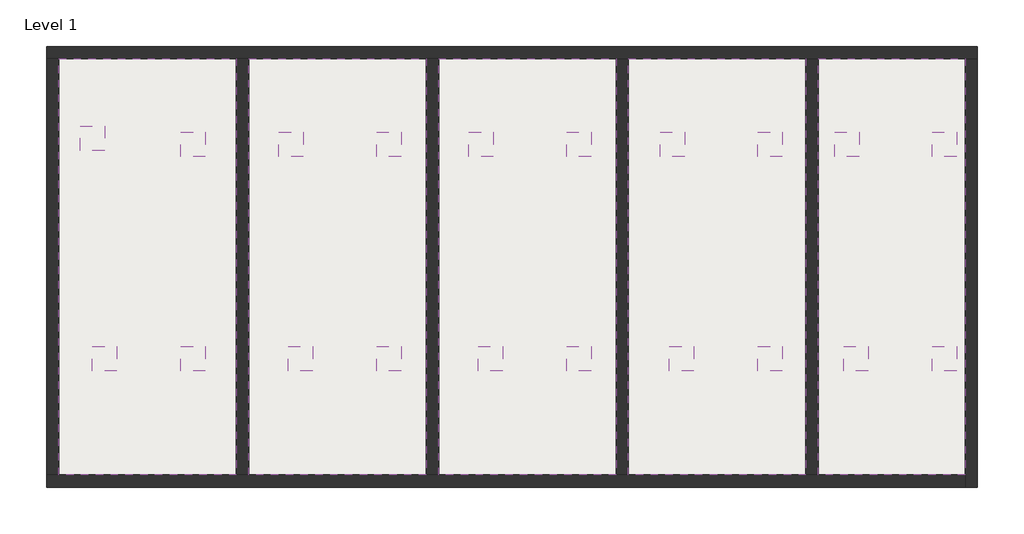
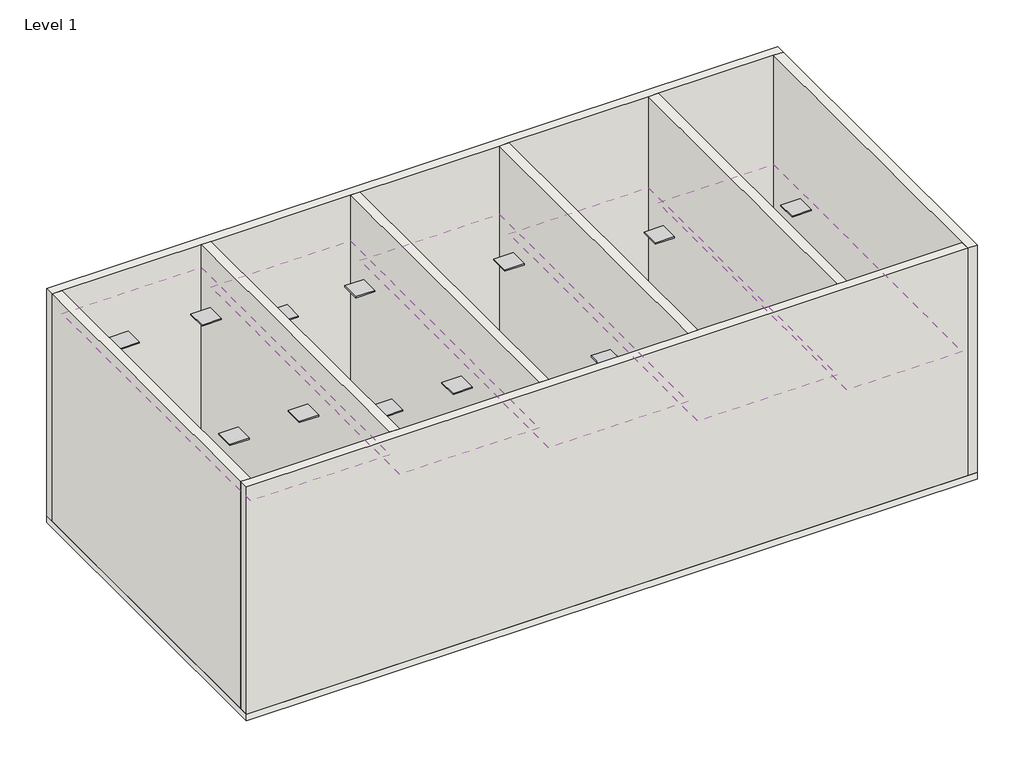
# One storey: 20 light fixtures, 8 walls, 5 coverings, 1 slab.
"""IFC4 building model written with IfcOpenShell, lengths in millimetres."""

import ifcopenshell
import ifcopenshell.guid

model = None  # the IFC model being written
_history = None  # IfcOwnerHistory: only IFC2X3 demands one
_inside = {}  # id of a spatial element -> (the spatial element, [elements in it])
_under = {}  # id of a project, library or spatial element -> (it, [spatial elements below it])
_declared = {}  # id of a project -> (the project, [libraries it declares])
_typed = {}  # id of a type object -> (the type object, [elements of that type])
_made_of = {}  # id of a material, layer set ... -> (it, [elements and type objects made of it])


def new_model(schema):
    """Start an empty IFC model of exactly this schema.

    Asked for "IFC4X3", IfcOpenShell would pick the latest addendum, in which some entities
    have other attributes; the version numbers below select the first issue.
    IFC2X3 requires an IfcOwnerHistory on every rooted entity: one is made here for all.
    """
    global model, _history
    if schema == "IFC4X3":
        model = ifcopenshell.file(schema_version=(4, 3, 0, 0))
    else:
        model = ifcopenshell.file(schema=schema)
    _inside.clear()
    _under.clear()
    _declared.clear()
    _typed.clear()
    _made_of.clear()
    _history = None
    if model.schema == "IFC2X3":
        org = make("IfcOrganization", Name="unknown")
        user = make(
            "IfcPersonAndOrganization",
            ThePerson=make("IfcPerson", FamilyName="unknown"),
            TheOrganization=org,
        )
        app = make(
            "IfcApplication",
            ApplicationDeveloper=org,
            Version="unknown",
            ApplicationFullName="unknown",
            ApplicationIdentifier="unknown",
        )
        _history = make(
            "IfcOwnerHistory",
            OwningUser=user,
            OwningApplication=app,
            ChangeAction="ADDED",
            CreationDate=0,
        )
    return model


def make(cls, **values):
    """One entity of the class cls with the attributes given. An attribute that is None is left unset."""
    return model.create_entity(
        cls, **{name: value for name, value in values.items() if value is not None}
    )


def rooted(cls, **values):
    """An entity with a GlobalId (a new one), such as an element, a storey or a relation."""
    return make(cls, GlobalId=ifcopenshell.guid.new(), OwnerHistory=_history, **values)


def si_unit(unit_type, name, prefix=None):
    """IfcSIUnit, for example si_unit("LENGTHUNIT", "METRE", prefix="MILLI")."""
    return make("IfcSIUnit", UnitType=unit_type, Prefix=prefix, Name=name)


def assignment(units):
    """IfcUnitAssignment: the units of a project."""
    return None if units is None else make("IfcUnitAssignment", Units=units)


def point(xyz):
    """IfcCartesianPoint."""
    return None if xyz is None else make("IfcCartesianPoint", Coordinates=xyz)


def direction(xyz):
    """IfcDirection."""
    return None if xyz is None else make("IfcDirection", DirectionRatios=xyz)


def frame(location, z_axis=None, x_axis=None):
    """IfcAxis2Placement3D, a coordinate frame: its origin and axes. An axis left out is left unset."""
    return make(
        "IfcAxis2Placement3D",
        Location=point(location),
        Axis=direction(z_axis),
        RefDirection=direction(x_axis),
    )


def origin():
    """The frame at (0, 0, 0) with its axes left unset."""
    return frame((0.0, 0.0, 0.0))


def origin_with_axes():
    """The frame at (0, 0, 0) with the z axis (0, 0, 1) and the x axis (1, 0, 0) written out."""
    return frame((0.0, 0.0, 0.0), z_axis=(0.0, 0.0, 1.0), x_axis=(1.0, 0.0, 0.0))


def place(relative_to, where):
    """IfcLocalPlacement: puts the frame where relative to a parent placement (None: the world)."""
    return make(
        "IfcLocalPlacement", PlacementRelTo=relative_to, RelativePlacement=where
    )


def context(
    kind, dimensions, precision=None, world=None, true_north=None, identifier=None
):
    """IfcGeometricRepresentationContext, for example the 3D "Model" context."""
    return make(
        "IfcGeometricRepresentationContext",
        ContextIdentifier=identifier,
        ContextType=kind,
        CoordinateSpaceDimension=dimensions,
        Precision=precision,
        WorldCoordinateSystem=world,
        TrueNorth=true_north,
    )


def project(units=None, contexts=None):
    """IfcProject with its units and contexts."""
    return rooted(
        "IfcProject",
        Name="project",
        RepresentationContexts=contexts,
        UnitsInContext=assignment(units),
    )


def spatial(cls, under=None, at=None, **own):
    """A site, building, storey or space (cls), placed at a placement, below another one or the project."""
    s = rooted(cls, ObjectPlacement=at, **own)
    if under is not None:
        _under.setdefault(under.id(), (under, []))[1].append(s)
    return s


def polyline(points):
    """IfcPolyline through the points."""
    return make("IfcPolyline", Points=[point(p) for p in points])


def outline(outer, holes=None, kind="AREA"):
    """IfcArbitraryClosedProfileDef: a profile drawn as a closed curve; with holes, ...WithVoids."""
    if holes is None:
        return make("IfcArbitraryClosedProfileDef", ProfileType=kind, OuterCurve=outer)
    return make(
        "IfcArbitraryProfileDefWithVoids",
        ProfileType=kind,
        OuterCurve=outer,
        InnerCurves=holes,
    )


def extrude(swept, where, along, depth):
    """IfcExtrudedAreaSolid: the profile swept, set in the frame where, extruded along a direction by depth."""
    return make(
        "IfcExtrudedAreaSolid",
        SweptArea=swept,
        Position=where,
        ExtrudedDirection=direction(along),
        Depth=depth,
    )


def faces_of(points, faces, orient=None, outer=None):
    """IfcFace entities. A face is a list of loops; a loop is a list of indices into points, from 0.

    orient and outer hold one flag for each loop. By default every Orientation is true, the
    first loop of a face is its IfcFaceOuterBound and the others are IfcFaceBound.
    """
    made = []
    for i, loops in enumerate(faces):
        bounds = []
        for j, loop in enumerate(loops):
            is_outer = j == 0 if outer is None else outer[i][j]
            bounds.append(
                make(
                    "IfcFaceOuterBound" if is_outer else "IfcFaceBound",
                    Bound=make("IfcPolyLoop", Polygon=[points[k] for k in loop]),
                    Orientation=True if orient is None else orient[i][j],
                )
            )
        made.append(make("IfcFace", Bounds=bounds))
    return made


def faceted_brep(points, faces, orient=None, outer=None, voids=None):
    """IfcFacetedBrep: a solid bounded by flat faces; with voids (closed shells), ...WithVoids."""
    shared = [point(p) for p in points]
    hull = make("IfcClosedShell", CfsFaces=faces_of(shared, faces, orient, outer))
    if voids is None:
        return make("IfcFacetedBrep", Outer=hull)
    return make(
        "IfcFacetedBrepWithVoids",
        Outer=hull,
        Voids=[
            make(cls, CfsFaces=faces_of(shared, fs, o, b)) for cls, fs, o, b in voids
        ],
    )


def shape(context_of_items, identifier, shape_type, items):
    """IfcShapeRepresentation: the items that make up one representation, for example the "Body"."""
    return make(
        "IfcShapeRepresentation",
        ContextOfItems=context_of_items,
        RepresentationIdentifier=identifier,
        RepresentationType=shape_type,
        Items=items,
    )


def source(mapping_origin, context_of_items, identifier, shape_type, items):
    """IfcRepresentationMap: a shape defined once, which mapped items show again and again."""
    return make(
        "IfcRepresentationMap",
        MappingOrigin=mapping_origin,
        MappedRepresentation=shape(context_of_items, identifier, shape_type, items),
    )


def transform(
    local_origin,
    x_axis=None,
    y_axis=None,
    z_axis=None,
    scale=None,
    scale2=None,
    scale3=None,
    uniform=True,
):
    """IfcCartesianTransformationOperator3D, or its non-uniform kind. x_axis, y_axis, z_axis: its Axis1, 2, 3."""
    if uniform:
        return make(
            "IfcCartesianTransformationOperator3D",
            Axis1=direction(x_axis),
            Axis2=direction(y_axis),
            LocalOrigin=point(local_origin),
            Scale=scale,
            Axis3=direction(z_axis),
        )
    return make(
        "IfcCartesianTransformationOperator3DnonUniform",
        Axis1=direction(x_axis),
        Axis2=direction(y_axis),
        LocalOrigin=point(local_origin),
        Scale=scale,
        Axis3=direction(z_axis),
        Scale2=scale2,
        Scale3=scale3,
    )


def mapped(mapping_source, mapping_target):
    """IfcMappedItem: shows the shape of a source again, moved by a transform."""
    return make(
        "IfcMappedItem", MappingSource=mapping_source, MappingTarget=mapping_target
    )


def made_of(thing, what):
    """Note that an element or type object is made of a material, layer set ...; save() writes the relation."""
    if what is not None:
        _made_of.setdefault(what.id(), (what, []))[1].append(thing)
    return thing


def element(
    cls,
    number,
    at=None,
    inside=None,
    cuts=None,
    type_object=None,
    material=None,
    context=None,
    identifier="Body",
    shape_type=None,
    held_by="IfcProductDefinitionShape",
    body=None,
    shapes=None,
    **own,
):
    """One element of the class cls, such as IfcWall. Its Tag is "e" and its number.

    at: its placement. inside: the storey or other place that contains it. cuts: it is an
    opening in that element (IfcRelVoidsElement). A single representation is given by context,
    identifier, shape_type and body (its items); several are given by shapes. held_by: the class
    of the entity that holds the representations. save() writes the other relations.
    """
    e = rooted(cls, Tag="e%d" % number, ObjectPlacement=at, **own)
    if body is not None:
        shapes = [shape(context, identifier, shape_type, body)]
    if shapes is not None:
        e.Representation = make(held_by, Representations=shapes)
    if inside is not None:
        _inside.setdefault(inside.id(), (inside, []))[1].append(e)
    if cuts is not None:
        rooted(
            "IfcRelVoidsElement", RelatingBuildingElement=cuts, RelatedOpeningElement=e
        )
    if type_object is not None:
        _typed.setdefault(type_object.id(), (type_object, []))[1].append(e)
    return made_of(e, material)


def aggregate(whole, parts):
    """IfcRelAggregates: a whole, such as a stair, and the parts it consists of."""
    return rooted("IfcRelAggregates", RelatingObject=whole, RelatedObjects=parts)


def save(model, path):
    """Write the relations noted so far, then the file.

    IfcRelAggregates (storeys below a building ...), IfcRelContainedInSpatialStructure (elements
    in a storey), IfcRelDefinesByType, IfcRelAssociatesMaterial and IfcRelDeclares: one each for
    every whole, place, type object, material and project.
    """
    for whole, parts in _under.values():
        aggregate(whole, parts)
    for where, things in _inside.values():
        rooted(
            "IfcRelContainedInSpatialStructure",
            RelatedElements=things,
            RelatingStructure=where,
        )
    for kind, things in _typed.values():
        rooted("IfcRelDefinesByType", RelatedObjects=things, RelatingType=kind)
    for what, things in _made_of.values():
        rooted("IfcRelAssociatesMaterial", RelatedObjects=things, RelatingMaterial=what)
    for by, libraries in _declared.values():
        rooted("IfcRelDeclares", RelatingContext=by, RelatedDefinitions=libraries)
    model.write(path)


def downlight_downlight_20077eaa(model_context):
    return source(origin(), model_context, "Body", "SweptSolid", [
        extrude(outline(polyline([(200.0, -200.0), (-200.0, -200.0), (-200.0, 200.0), (200.0, 200.0), (200.0, -200.0)])), frame((0.0, 0.0, -4.6872227), z_axis=(0.0, 0.0, 1.0), x_axis=(1.0, 0.0, 0.0)), (0.0, 0.0, 1.0), 24.9370919),
    ])


model = new_model("IFC4")

# Units and contexts
model_context = context("Model", 3, world=origin())
ifc_project = project(units=[si_unit("LENGTHUNIT", "METRE", prefix="MILLI")], contexts=[model_context])

# Site, building, storey
site = spatial("IfcSite", under=ifc_project)
building = spatial("IfcBuilding", under=site)
storey = spatial("IfcBuildingStorey", under=building, Name="Level 1", Elevation=0.0)

# Coverings
placement = place(None, origin())
element("IfcCovering", 1, ObjectType="600 x 600mm Grid", at=placement, inside=storey, context=model_context, shape_type="SweptSolid", body=[
    extrude(outline(polyline([(4711.6370984, -2494.7382368), (4711.6370984, 4305.2617632), (7111.6370984, 4305.2617632), (7111.6370984, -2494.7382368), (4711.6370984, -2494.7382368)])), frame((0.0, 0.0, 2600.0), z_axis=(0.0, 0.0, 1.0), x_axis=(1.0, 0.0, 0.0)), (0.0, 0.0, 1.0), 52.0),
])
element("IfcCovering", 2, ObjectType="600 x 600mm Grid", at=placement, inside=storey, context=model_context, shape_type="SweptSolid", body=[
    extrude(outline(polyline([(1611.6370984, -2494.7382368), (1611.6370984, 4305.2617632), (4511.6370984, 4305.2617632), (4511.6370984, -2494.7382368), (1611.6370984, -2494.7382368)])), frame((0.0, 0.0, 3000.0), z_axis=(0.0, 0.0, 1.0), x_axis=(1.0, 0.0, 0.0)), (0.0, 0.0, 1.0), 52.0),
])
element("IfcCovering", 3, ObjectType="600 x 600mm Grid", at=placement, inside=storey, context=model_context, shape_type="SweptSolid", body=[
    extrude(outline(polyline([(-1488.3629016, -2494.7382368), (-1488.3629016, 4305.2617632), (1411.6370984, 4305.2617632), (1411.6370984, -2494.7382368), (-1488.3629016, -2494.7382368)])), frame((0.0, 0.0, 3500.0), z_axis=(0.0, 0.0, 1.0), x_axis=(1.0, 0.0, 0.0)), (0.0, 0.0, 1.0), 52.0),
])
element("IfcCovering", 4, ObjectType="600 x 600mm Grid", at=placement, inside=storey, context=model_context, shape_type="SweptSolid", body=[
    extrude(outline(polyline([(-4588.3629016, -2494.7382368), (-4588.3629016, 4305.2617632), (-1688.3629016, 4305.2617632), (-1688.3629016, -2494.7382368), (-4588.3629016, -2494.7382368)])), frame((0.0, 0.0, 4000.0), z_axis=(0.0, 0.0, 1.0), x_axis=(1.0, 0.0, 0.0)), (0.0, 0.0, 1.0), 52.0),
])
element("IfcCovering", 5, ObjectType="600 x 600mm Grid", at=placement, inside=storey, context=model_context, shape_type="SweptSolid", body=[
    extrude(outline(polyline([(-7688.3629016, 4305.2617632), (-4788.3629016, 4305.2617632), (-4788.3629016, -2494.7382368), (-7688.3629016, -2494.7382368), (-7688.3629016, 4305.2617632)])), frame((0.0, 0.0, 4500.0), z_axis=(0.0, 0.0, 1.0), x_axis=(1.0, 0.0, 0.0)), (0.0, 0.0, 1.0), 52.0),
])

# Light fixtures
downlight_downlight_shape = downlight_downlight_20077eaa(model_context)
element("IfcLightFixture", 6, ObjectType="Downlight : Downlight", at=placement, inside=storey, context=model_context, shape_type="MappedRepresentation", body=[
    mapped(downlight_downlight_shape, transform((-7138.3629016, 3005.2617632, 4500.0), x_axis=(1.0, 0.0, 0.0), y_axis=(0.0, 1.0, 0.0), z_axis=(0.0, 0.0, 1.0))),
])
element("IfcLightFixture", 7, ObjectType="Downlight : Downlight", at=placement, inside=storey, context=model_context, shape_type="MappedRepresentation", body=[
    mapped(downlight_downlight_shape, transform((-5493.1629016, 2905.2617632, 4500.0), x_axis=(1.0, 0.0, 0.0), y_axis=(0.0, 1.0, 0.0), z_axis=(0.0, 0.0, 1.0))),
])
element("IfcLightFixture", 8, ObjectType="Downlight : Downlight", at=placement, inside=storey, context=model_context, shape_type="MappedRepresentation", body=[
    mapped(downlight_downlight_shape, transform((-5493.1629016, -599.5382368, 4500.0), x_axis=(1.0, 0.0, 0.0), y_axis=(0.0, 1.0, 0.0), z_axis=(0.0, 0.0, 1.0))),
])
element("IfcLightFixture", 9, ObjectType="Downlight : Downlight", at=placement, inside=storey, context=model_context, shape_type="MappedRepresentation", body=[
    mapped(downlight_downlight_shape, transform((-6938.3629016, -599.5382368, 4500.0), x_axis=(1.0, 0.0, 0.0), y_axis=(0.0, 1.0, 0.0), z_axis=(0.0, 0.0, 1.0))),
])
element("IfcLightFixture", 10, ObjectType="Downlight : Downlight", at=placement, inside=storey, context=model_context, shape_type="MappedRepresentation", body=[
    mapped(downlight_downlight_shape, transform((-3893.1629016, 2905.2617632, 4000.0), x_axis=(1.0, 0.0, 0.0), y_axis=(0.0, 1.0, 0.0), z_axis=(0.0, 0.0, 1.0))),
])
element("IfcLightFixture", 11, ObjectType="Downlight : Downlight", at=placement, inside=storey, context=model_context, shape_type="MappedRepresentation", body=[
    mapped(downlight_downlight_shape, transform((-2297.9629016, 2905.2617632, 4000.0), x_axis=(1.0, 0.0, 0.0), y_axis=(0.0, 1.0, 0.0), z_axis=(0.0, 0.0, 1.0))),
])
element("IfcLightFixture", 12, ObjectType="Downlight : Downlight", at=placement, inside=storey, context=model_context, shape_type="MappedRepresentation", body=[
    mapped(downlight_downlight_shape, transform((-2297.9629016, -599.5382368, 4000.0), x_axis=(1.0, 0.0, 0.0), y_axis=(0.0, 1.0, 0.0), z_axis=(0.0, 0.0, 1.0))),
])
element("IfcLightFixture", 13, ObjectType="Downlight : Downlight", at=placement, inside=storey, context=model_context, shape_type="MappedRepresentation", body=[
    mapped(downlight_downlight_shape, transform((-3743.1629016, -599.5382368, 4000.0), x_axis=(1.0, 0.0, 0.0), y_axis=(0.0, 1.0, 0.0), z_axis=(0.0, 0.0, 1.0))),
])
element("IfcLightFixture", 14, ObjectType="Downlight : Downlight", at=placement, inside=storey, context=model_context, shape_type="MappedRepresentation", body=[
    mapped(downlight_downlight_shape, transform((-790.9030237, 2905.2617632, 3500.0), x_axis=(1.0, 0.0, 0.0), y_axis=(0.0, 1.0, 0.0), z_axis=(0.0, 0.0, 1.0))),
])
element("IfcLightFixture", 15, ObjectType="Downlight : Downlight", at=placement, inside=storey, context=model_context, shape_type="MappedRepresentation", body=[
    mapped(downlight_downlight_shape, transform((804.2969763, 2905.2617632, 3500.0), x_axis=(1.0, 0.0, 0.0), y_axis=(0.0, 1.0, 0.0), z_axis=(0.0, 0.0, 1.0))),
])
element("IfcLightFixture", 16, ObjectType="Downlight : Downlight", at=placement, inside=storey, context=model_context, shape_type="MappedRepresentation", body=[
    mapped(downlight_downlight_shape, transform((804.2969763, -599.5382368, 3500.0), x_axis=(1.0, 0.0, 0.0), y_axis=(0.0, 1.0, 0.0), z_axis=(0.0, 0.0, 1.0))),
])
element("IfcLightFixture", 17, ObjectType="Downlight : Downlight", at=placement, inside=storey, context=model_context, shape_type="MappedRepresentation", body=[
    mapped(downlight_downlight_shape, transform((-640.9030237, -599.5382368, 3500.0), x_axis=(1.0, 0.0, 0.0), y_axis=(0.0, 1.0, 0.0), z_axis=(0.0, 0.0, 1.0))),
])
element("IfcLightFixture", 18, ObjectType="Downlight : Downlight", at=placement, inside=storey, context=model_context, shape_type="MappedRepresentation", body=[
    mapped(downlight_downlight_shape, transform((2331.8395219, 2905.2617632, 3000.0), x_axis=(1.0, 0.0, 0.0), y_axis=(0.0, 1.0, 0.0), z_axis=(0.0, 0.0, 1.0))),
])
element("IfcLightFixture", 19, ObjectType="Downlight : Downlight", at=placement, inside=storey, context=model_context, shape_type="MappedRepresentation", body=[
    mapped(downlight_downlight_shape, transform((3927.0395219, 2905.2617632, 3000.0), x_axis=(1.0, 0.0, 0.0), y_axis=(0.0, 1.0, 0.0), z_axis=(0.0, 0.0, 1.0))),
])
element("IfcLightFixture", 20, ObjectType="Downlight : Downlight", at=placement, inside=storey, context=model_context, shape_type="MappedRepresentation", body=[
    mapped(downlight_downlight_shape, transform((3927.0395219, -599.5382368, 3000.0), x_axis=(1.0, 0.0, 0.0), y_axis=(0.0, 1.0, 0.0), z_axis=(0.0, 0.0, 1.0))),
])
element("IfcLightFixture", 21, ObjectType="Downlight : Downlight", at=placement, inside=storey, context=model_context, shape_type="MappedRepresentation", body=[
    mapped(downlight_downlight_shape, transform((2481.8395219, -599.5382368, 3000.0), x_axis=(1.0, 0.0, 0.0), y_axis=(0.0, 1.0, 0.0), z_axis=(0.0, 0.0, 1.0))),
])
element("IfcLightFixture", 22, ObjectType="Downlight : Downlight", at=placement, inside=storey, context=model_context, shape_type="MappedRepresentation", body=[
    mapped(downlight_downlight_shape, transform((5177.9874108, 2905.2617632, 2600.0), x_axis=(1.0, 0.0, 0.0), y_axis=(0.0, 1.0, 0.0), z_axis=(0.0, 0.0, 1.0))),
])
element("IfcLightFixture", 23, ObjectType="Downlight : Downlight", at=placement, inside=storey, context=model_context, shape_type="MappedRepresentation", body=[
    mapped(downlight_downlight_shape, transform((6773.1874108, 2905.2617632, 2600.0), x_axis=(1.0, 0.0, 0.0), y_axis=(0.0, 1.0, 0.0), z_axis=(0.0, 0.0, 1.0))),
])
element("IfcLightFixture", 24, ObjectType="Downlight : Downlight", at=placement, inside=storey, context=model_context, shape_type="MappedRepresentation", body=[
    mapped(downlight_downlight_shape, transform((6773.1874108, -599.5382368, 2600.0), x_axis=(1.0, 0.0, 0.0), y_axis=(0.0, 1.0, 0.0), z_axis=(0.0, 0.0, 1.0))),
])
element("IfcLightFixture", 25, ObjectType="Downlight : Downlight", at=placement, inside=storey, context=model_context, shape_type="MappedRepresentation", body=[
    mapped(downlight_downlight_shape, transform((5327.9874108, -599.5382368, 2600.0), x_axis=(1.0, 0.0, 0.0), y_axis=(0.0, 1.0, 0.0), z_axis=(0.0, 0.0, 1.0))),
])

# Slab
element("IfcSlab", 26, ObjectType="Generic 150mm", at=placement, inside=storey, context=model_context, shape_type="SweptSolid", body=[
    extrude(outline(polyline([(7311.6370984, 4505.2617632), (7311.6370984, -2694.7382368), (-7888.3629016, -2694.7382368), (-7888.3629016, 4505.2617632), (7311.6370984, 4505.2617632)])), frame((0.0, 0.0, -150.0), z_axis=(0.0, 0.0, 1.0), x_axis=(1.0, 0.0, 0.0)), (0.0, 0.0, 1.0), 150.0),
])

# Walls
element("IfcWall", 27, ObjectType="Generic - 200mm", at=placement, inside=storey, context=model_context, shape_type="Brep", body=[
    faceted_brep([(-7888.3629016, 4305.2617632, 0.0), (-7688.3629016, 4305.2617632, 0.0), (-4788.3629016, 4305.2617632, 0.0), (-4588.3629016, 4305.2617632, 0.0), (-1688.3629016, 4305.2617632, 0.0), (-1488.3629016, 4305.2617632, 0.0), (1411.6370984, 4305.2617632, 0.0), (1611.6370984, 4305.2617632, 0.0), (4511.6370984, 4305.2617632, 0.0), (4711.6370984, 4305.2617632, 0.0), (7111.6370984, 4305.2617632, 0.0), (7311.6370984, 4305.2617632, 0.0), (7311.6370984, 4305.2617632, 5000.0), (7111.6370984, 4305.2617632, 5000.0), (4711.6370984, 4305.2617632, 5000.0), (4511.6370984, 4305.2617632, 5000.0), (1611.6370984, 4305.2617632, 5000.0), (1411.6370984, 4305.2617632, 5000.0), (-1488.3629016, 4305.2617632, 5000.0), (-1688.3629016, 4305.2617632, 5000.0), (-4588.3629016, 4305.2617632, 5000.0), (-4788.3629016, 4305.2617632, 5000.0), (-7688.3629016, 4305.2617632, 5000.0), (-7888.3629016, 4305.2617632, 5000.0), (-7888.3629016, 4505.2617632, 0.0), (-7888.3629016, 4505.2617632, 5000.0), (7311.6370984, 4505.2617632, 5000.0), (7311.6370984, 4505.2617632, 0.0)], [[[0, 1, 2, 3, 4, 5, 6, 7, 8, 9, 10, 11, 12, 13, 14, 15, 16, 17, 18, 19, 20, 21, 22, 23]], [[24, 25, 26, 27]], [[11, 10, 9, 8, 7, 6, 5, 4, 3, 2, 1, 0, 24, 27]], [[23, 22, 21, 20, 19, 18, 17, 16, 15, 14, 13, 12, 26, 25]], [[12, 11, 27, 26]], [[0, 23, 25, 24]]]),
])
element("IfcWall", 28, ObjectType="Generic - 200mm", at=placement, inside=storey, context=model_context, shape_type="Brep", body=[
    faceted_brep([(7111.6370984, 4305.2617632, 0.0), (7111.6370984, -2494.7382368, 0.0), (7111.6370984, -2694.7382368, 0.0), (7111.6370984, -2694.7382368, 5000.0), (7111.6370984, -2494.7382368, 5000.0), (7111.6370984, 4305.2617632, 5000.0), (7311.6370984, 4305.2617632, 0.0), (7311.6370984, 4305.2617632, 5000.0), (7311.6370984, -2694.7382368, 5000.0), (7311.6370984, -2694.7382368, 0.0)], [[[0, 1, 2, 3, 4, 5]], [[6, 7, 8, 9]], [[2, 1, 0, 6, 9]], [[5, 4, 3, 8, 7]], [[0, 5, 7, 6]], [[3, 2, 9, 8]]]),
])
element("IfcWall", 29, ObjectType="Generic - 200mm", at=placement, inside=storey, context=model_context, shape_type="Brep", body=[
    faceted_brep([(7111.6370984, -2494.7382368, 0.0), (4711.6370984, -2494.7382368, 0.0), (4511.6370984, -2494.7382368, 0.0), (1611.6370984, -2494.7382368, 0.0), (1411.6370984, -2494.7382368, 0.0), (-1488.3629016, -2494.7382368, 0.0), (-1688.3629016, -2494.7382368, 0.0), (-4588.3629016, -2494.7382368, 0.0), (-4788.3629016, -2494.7382368, 0.0), (-7688.3629016, -2494.7382368, 0.0), (-7888.3629016, -2494.7382368, 0.0), (-7888.3629016, -2494.7382368, 5000.0), (-7688.3629016, -2494.7382368, 5000.0), (-4788.3629016, -2494.7382368, 5000.0), (-4588.3629016, -2494.7382368, 5000.0), (-1688.3629016, -2494.7382368, 5000.0), (-1488.3629016, -2494.7382368, 5000.0), (1411.6370984, -2494.7382368, 5000.0), (1611.6370984, -2494.7382368, 5000.0), (4511.6370984, -2494.7382368, 5000.0), (4711.6370984, -2494.7382368, 5000.0), (7111.6370984, -2494.7382368, 5000.0), (7111.6370984, -2694.7382368, 0.0), (7111.6370984, -2694.7382368, 5000.0), (-7888.3629016, -2694.7382368, 5000.0), (-7888.3629016, -2694.7382368, 0.0)], [[[0, 1, 2, 3, 4, 5, 6, 7, 8, 9, 10, 11, 12, 13, 14, 15, 16, 17, 18, 19, 20, 21]], [[22, 23, 24, 25]], [[10, 9, 8, 7, 6, 5, 4, 3, 2, 1, 0, 22, 25]], [[21, 20, 19, 18, 17, 16, 15, 14, 13, 12, 11, 24, 23]], [[0, 21, 23, 22]], [[11, 10, 25, 24]]]),
])
element("IfcWall", 30, ObjectType="Generic - 200mm", at=placement, inside=storey, context=model_context, shape_type="SweptSolid", body=[
    extrude(outline(polyline([(-7688.3629016, 4305.2617632), (-7688.3629016, -2494.7382368), (-7888.3629016, -2494.7382368), (-7888.3629016, 4305.2617632), (-7688.3629016, 4305.2617632)])), origin_with_axes(), (0.0, 0.0, 1.0), 5000.0),
])
element("IfcWall", 31, ObjectType="Generic - 200mm", at=placement, inside=storey, context=model_context, shape_type="SweptSolid", body=[
    extrude(outline(polyline([(-4788.3629016, -2494.7382368), (-4788.3629016, 4305.2617632), (-4588.3629016, 4305.2617632), (-4588.3629016, -2494.7382368), (-4788.3629016, -2494.7382368)])), origin_with_axes(), (0.0, 0.0, 1.0), 5000.0),
])
element("IfcWall", 32, ObjectType="Generic - 200mm", at=placement, inside=storey, context=model_context, shape_type="SweptSolid", body=[
    extrude(outline(polyline([(-1688.3629016, -2494.7382368), (-1688.3629016, 4305.2617632), (-1488.3629016, 4305.2617632), (-1488.3629016, -2494.7382368), (-1688.3629016, -2494.7382368)])), origin_with_axes(), (0.0, 0.0, 1.0), 5000.0),
])
element("IfcWall", 33, ObjectType="Generic - 200mm", at=placement, inside=storey, context=model_context, shape_type="SweptSolid", body=[
    extrude(outline(polyline([(1411.6370984, -2494.7382368), (1411.6370984, 4305.2617632), (1611.6370984, 4305.2617632), (1611.6370984, -2494.7382368), (1411.6370984, -2494.7382368)])), origin_with_axes(), (0.0, 0.0, 1.0), 5000.0),
])
element("IfcWall", 34, ObjectType="Generic - 200mm", at=placement, inside=storey, context=model_context, shape_type="SweptSolid", body=[
    extrude(outline(polyline([(4511.6370984, -2494.7382368), (4511.6370984, 4305.2617632), (4711.6370984, 4305.2617632), (4711.6370984, -2494.7382368), (4511.6370984, -2494.7382368)])), origin_with_axes(), (0.0, 0.0, 1.0), 5000.0),
])

save(model, "model.ifc")

# Revit data of these elements
# Project information
#   Project Issue Date = "Issue Date"
#   Project Status = "Project Status"
#   Client Name = "Owner"
#   Project Address = "Enter address here"
#   Project Name = "Project Name"
#   Project Number = "0001"
# Type "600 x 600mm Grid"
#   built-in parameter 1002203 = 1 (stored number, unit not read)
#   built-in parameter 1002202 = 1 (stored number, unit not read)
#   Layers, outside or top first: 0.036 m "Default" (function 1); 0.016 m "Ceiling Tile 600 x 600" (function 5)
# Type "Downlight : Downlight"
#   Default Elevation = 0
# Type "Generic 150mm"
#   Function = 0
#   Layers, outside or top first: 0.15 m no material (function 1)
# Type "Generic - 200mm"
#   Layers, outside or top first: 0.2 m no material (function 1)
# Element 1 (IfcCovering, "600 x 600mm Grid")
#   Height Offset From Level = 2.6 m
#   Phase Created = New Construction
#   Materials on its faces: "Ceiling Tile 600 x 600", "Default"
# Element 2 (IfcCovering, "600 x 600mm Grid")
#   Height Offset From Level = 3 m
#   Phase Created = New Construction
#   Materials on its faces: "Ceiling Tile 600 x 600", "Default"
# Element 3 (IfcCovering, "600 x 600mm Grid")
#   Height Offset From Level = 3.5 m
#   Phase Created = New Construction
#   Materials on its faces: "Ceiling Tile 600 x 600", "Default"
# Element 4 (IfcCovering, "600 x 600mm Grid")
#   Height Offset From Level = 4 m
#   Phase Created = New Construction
#   Materials on its faces: "Ceiling Tile 600 x 600", "Default"
# Element 5 (IfcCovering, "600 x 600mm Grid")
#   Height Offset From Level = 4.5 m
#   Phase Created = New Construction
#   Materials on its faces: "Ceiling Tile 600 x 600", "Default"
# Element 6 (IfcLightFixture, "Downlight : Downlight")
#   Mark = "24"
#   Phase Created = New Construction
# Element 7 (IfcLightFixture, "Downlight : Downlight")
#   Mark = "55"
#   Phase Created = New Construction
# Element 8 (IfcLightFixture, "Downlight : Downlight")
#   Mark = "56"
#   Phase Created = New Construction
# Element 9 (IfcLightFixture, "Downlight : Downlight")
#   Mark = "57"
#   Phase Created = New Construction
# Element 10 (IfcLightFixture, "Downlight : Downlight")
#   Mark = "58"
#   Phase Created = New Construction
# Element 11 (IfcLightFixture, "Downlight : Downlight")
#   Mark = "59"
#   Phase Created = New Construction
# Element 12 (IfcLightFixture, "Downlight : Downlight")
#   Mark = "60"
#   Phase Created = New Construction
# Element 13 (IfcLightFixture, "Downlight : Downlight")
#   Mark = "61"
#   Phase Created = New Construction
# Element 14 (IfcLightFixture, "Downlight : Downlight")
#   Mark = "62"
#   Phase Created = New Construction
# Element 15 (IfcLightFixture, "Downlight : Downlight")
#   Mark = "63"
#   Phase Created = New Construction
# Element 16 (IfcLightFixture, "Downlight : Downlight")
#   Mark = "64"
#   Phase Created = New Construction
# Element 17 (IfcLightFixture, "Downlight : Downlight")
#   Mark = "65"
#   Phase Created = New Construction
# Element 18 (IfcLightFixture, "Downlight : Downlight")
#   Mark = "66"
#   Phase Created = New Construction
# Element 19 (IfcLightFixture, "Downlight : Downlight")
#   Mark = "67"
#   Phase Created = New Construction
# Element 20 (IfcLightFixture, "Downlight : Downlight")
#   Mark = "68"
#   Phase Created = New Construction
# Element 21 (IfcLightFixture, "Downlight : Downlight")
#   Mark = "69"
#   Phase Created = New Construction
# Element 22 (IfcLightFixture, "Downlight : Downlight")
#   Mark = "70"
#   Phase Created = New Construction
# Element 23 (IfcLightFixture, "Downlight : Downlight")
#   Mark = "71"
#   Phase Created = New Construction
# Element 24 (IfcLightFixture, "Downlight : Downlight")
#   Mark = "72"
#   Phase Created = New Construction
# Element 25 (IfcLightFixture, "Downlight : Downlight")
#   Mark = "73"
#   Phase Created = New Construction
# Element 26 (IfcSlab, "Generic 150mm")
#   Height Offset From Level = 0 m
#   Phase Created = New Construction
#   Materials on its faces: "Default Floor"
# Elements 27, 28, 29, 30, 31, 32, 33, 34 (IfcWall, "Generic - 200mm")
#   Top Offset = 0 m
#   Base Offset = 0 m
#   wall height = 5 m
#   Phase Created = New Construction
#   Base Constraint = Level 1
#   Top Constraint = Level 2
#   Materials on its faces: "Default Wall"
# Materials
#   "Default": class "Generic", colour RGB 127 127 127, transparency 0, Cost = 0
#   "Ceiling Tile 600 x 600": class "Generic", colour RGB 235 235 235, transparency 0, Description = "Acoustic ceiling tile", Cost = 0
#   "Default Floor": class "Miscellaneous", colour RGB 127 127 127, transparency 0, Cost = 0
#   "Default Wall": class "Miscellaneous", colour RGB 128 128 128, transparency 0, Cost = 0
